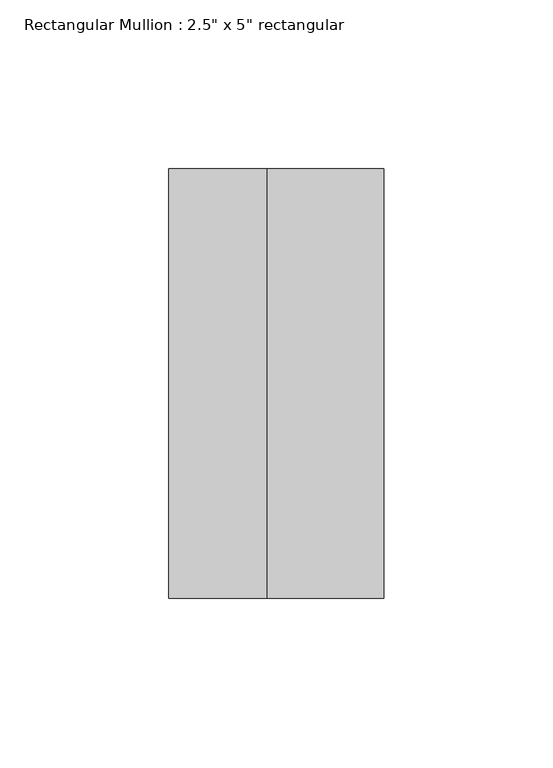
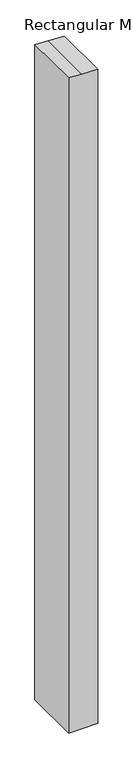
"""IFC4 building model written with IfcOpenShell, lengths in millimetres: member geometry."""

from ifc_helpers import new_model, si_unit, frame, origin, place, context, project, spatial, polyline, outline, extrude, source, transform, mapped, element, save


def member_5910e702(model_context):
    return source(origin(), model_context, "Body", "SweptSolid", [
        extrude(outline(polyline([(-64.8775557, 31.75), (-63.4449853, -2.6426951), (-62.232569, -31.75), (-1571.0379787, -31.75), (-1571.0379787, 31.75), (-64.8775557, 31.75)])), frame((0.0, -63.5, 0.0), z_axis=(0.0, 1.0, 0.0), x_axis=(0.0, 0.0, 1.0)), (0.0, 0.0, 1.0), 127.0),
    ])


if __name__ == "__main__":
    model = new_model("IFC4")
    model_context = context("Model", 3, world=origin())
    ifc_project = project(units=[si_unit("LENGTHUNIT", "METRE", prefix="MILLI")], contexts=[model_context])
    site = spatial("IfcSite", under=ifc_project)
    building = spatial("IfcBuilding", under=site)
    placement = place(None, origin())
    member_shape = member_5910e702(model_context)
    element("IfcMember", 1, ObjectType="Rectangular Mullion : 2.5\" x 5\" rectangular", at=placement, inside=building, context=model_context, shape_type="MappedRepresentation", body=[
        mapped(member_shape, transform((0.0, 0.0, 0.0), x_axis=(1.0, 0.0, 0.0), y_axis=(0.0, 1.0, 0.0), z_axis=(0.0, 0.0, 1.0))),
    ])
    save(model, "model.ifc")

# Revit data of these elements
# Type "Rectangular Mullion : 2.5\" x 5\" rectangular"
#   built-in parameter 1007304 = 0.416667 (stored number, unit not read)
#   built-in parameter 1007301 = 0.104167 (stored number, unit not read)
#   built-in parameter 1007300 = 0.104167 (stored number, unit not read)
# Element 1 (IfcMember, "Rectangular Mullion : 2.5\" x 5\" rectangular")
#   Materials on its faces: "Aluminum"
# Materials
#   "Aluminum": class "Metal", colour RGB 247 247 247, transparency 0, Description = "Aluminum 6061", Cost = 0
